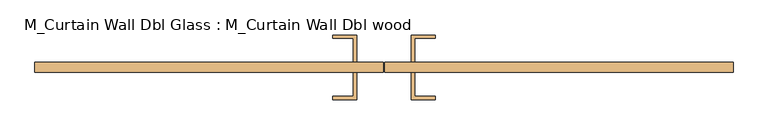
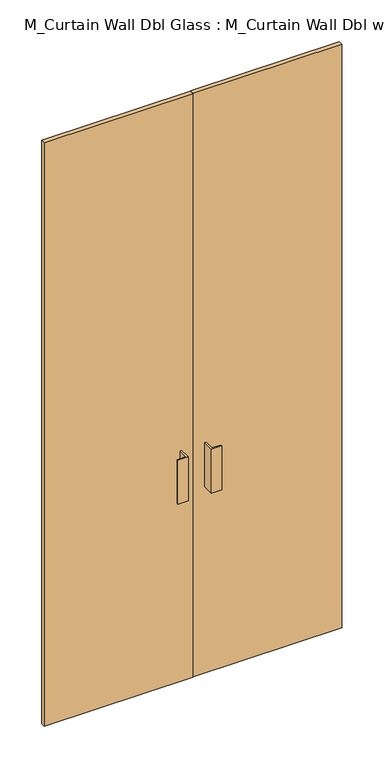
"""IFC4 building model written with IfcOpenShell, lengths in millimetres: door geometry, M_Curtain Wall Dbl Glass : M_Curtain Wall Dbl wood."""

from ifc_helpers import new_model, si_unit, frame, origin, origin_with_axes, place, context, project, spatial, polyline, outline, extrude, source, transform, mapped, element, save


def m_curtain_wall_dbl_glass_m_curtain_wall_dbl_wood_d0b68c61(model_context):
    return source(origin(), model_context, "Body", "SweptSolid", [
        extrude(outline(polyline([(-1.5875, 19.05), (-1.5875, 0.0), (-651.548373, 0.0), (-651.548373, 19.05), (-1.5875, 19.05)])), origin_with_axes(), (0.0, 0.0, 1.0), 2700.0),
        extrude(outline(polyline([(651.548373, 19.05), (651.548373, 0.0), (1.5875, 0.0), (1.5875, 19.05), (651.548373, 19.05)])), origin_with_axes(), (0.0, 0.0, 1.0), 2700.0),
        extrude(outline(polyline([(-50.8, -50.8), (-95.25, -50.8), (-95.25, -44.45), (-57.15, -44.45), (-57.15, 0.0), (-50.8, 0.0), (-50.8, -50.8)])), frame((0.0, 0.0, 863.6), z_axis=(0.0, 0.0, 1.0), x_axis=(1.0, 0.0, 0.0)), (0.0, 0.0, 1.0), 203.2),
        extrude(outline(polyline([(50.8, -50.8), (50.8, 0.0), (57.15, 0.0), (57.15, -44.45), (95.25, -44.45), (95.25, -50.8), (50.8, -50.8)])), frame((0.0, 0.0, 863.6), z_axis=(0.0, 0.0, 1.0), x_axis=(1.0, 0.0, 0.0)), (0.0, 0.0, 1.0), 203.2),
        extrude(outline(polyline([(-50.8, 69.85), (-50.8, 19.05), (-57.15, 19.05), (-57.15, 63.5), (-95.25, 63.5), (-95.25, 69.85), (-50.8, 69.85)])), frame((0.0, 0.0, 863.6), z_axis=(0.0, 0.0, 1.0), x_axis=(1.0, 0.0, 0.0)), (0.0, 0.0, 1.0), 203.2),
        extrude(outline(polyline([(50.8, 69.85), (95.25, 69.85), (95.25, 63.5), (57.15, 63.5), (57.15, 19.05), (50.8, 19.05), (50.8, 69.85)])), frame((0.0, 0.0, 863.6), z_axis=(0.0, 0.0, 1.0), x_axis=(1.0, 0.0, 0.0)), (0.0, 0.0, 1.0), 203.2),
    ])


if __name__ == "__main__":
    model = new_model("IFC4")
    model_context = context("Model", 3, world=origin())
    ifc_project = project(units=[si_unit("LENGTHUNIT", "METRE", prefix="MILLI")], contexts=[model_context])
    site = spatial("IfcSite", under=ifc_project)
    building = spatial("IfcBuilding", under=site)
    placement = place(None, origin())
    m_curtain_wall_dbl_glass_m_curtain_wall_dbl_wood_shape = m_curtain_wall_dbl_glass_m_curtain_wall_dbl_wood_d0b68c61(model_context)
    element("IfcDoor", 1, ObjectType="M_Curtain Wall Dbl Glass : M_Curtain Wall Dbl wood", at=placement, inside=building, context=model_context, shape_type="MappedRepresentation", body=[
        mapped(m_curtain_wall_dbl_glass_m_curtain_wall_dbl_wood_shape, transform((0.0, 0.0, 0.0), x_axis=(1.0, 0.0, 0.0), y_axis=(0.0, 1.0, 0.0), z_axis=(0.0, 0.0, 1.0))),
    ])
    save(model, "model.ifc")

# Revit data of these elements
# Type "M_Curtain Wall Dbl Glass : M_Curtain Wall Dbl wood"
#   Model = "12345679"
#   Manufacturer = "Dublin Doors"
#   Description = "Double Wood Door"
#   Type Mark = "46"
#   Fire Rating = "60M"
#   COBie.Type.CreatedBy = "design@eagle.com"
#   COBie.Type.CreatedOn = "2016-09-13T05:47:35"
#   COBie.Type.Name = "Doors_M_Curtain Wall Dbl Glass_M_Curtain Wall Dbl wood"
#   COBie.Type.Category = "23-30 10 00 : Doors"
#   COBie.Type.Description = "Double Wood Door"
#   COBie.Type.Manufacturer = "Dublin Doors"
#   COBie.Type.ModelNumber = "12345679"
#   Construction Type Id = "opn-d36"
#   Analytic Construction = "Wood panel"
#   COBie.Type.ReplacementCost = 0
#   Offset = 0 mm
#   Heat Transfer Coefficient (U) = 3.8042 W/(m²·K)
#   COBie.Type = yes
#   Function = 1
#   Glazing Material = Door - Panel
#   Visual Light Transmittance = 0
#   Solar Heat Gain Coefficient = 0
# Element 1 (IfcDoor, "M_Curtain Wall Dbl Glass : M_Curtain Wall Dbl wood")
#   Materials on its faces: "Aluminum", "Door - Panel"
# Materials
#   "Door - Panel": class "Wood", colour RGB 210 159 95, transparency 0
#   "Aluminum": class "Metal", colour RGB 247 247 247, transparency 0, Description = "Aluminum 6061", Cost = 0
